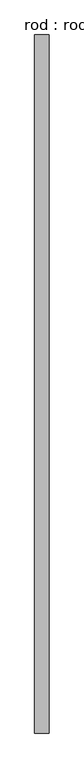
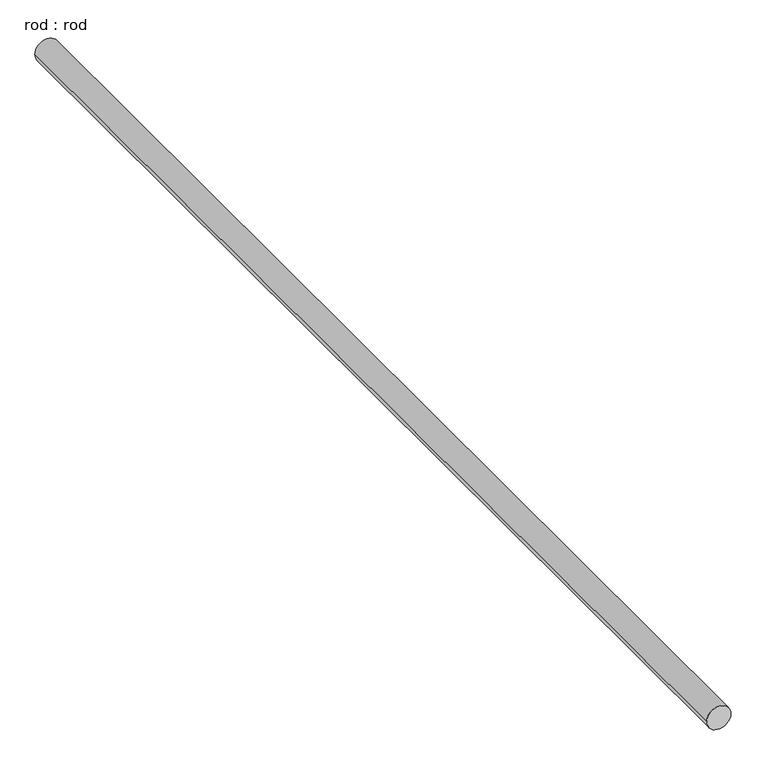
"""IFC4 building model written with IfcOpenShell, lengths in millimetres: proxy geometry, rod : rod."""

from ifc_helpers import new_model, si_unit, point, frame, frame_2d, origin, place, context, project, spatial, circle_curve, trimmed, segment, composite_curve, outline, extrude, source, transform, mapped, element, save


def rod_rod_0f7073d6(model_context):
    return source(origin(), model_context, "Body", "SweptSolid", [
        extrude(outline(composite_curve([segment(trimmed(circle_curve(frame_2d((0.0108462, 0.0)), 200.0), [point((0.0108462, 200.0))], [point((0.0108462, -200.0))], False, "CARTESIAN"), True, "CONTINUOUS"), segment(trimmed(circle_curve(frame_2d((0.0108462, 0.0)), 200.0), [point((0.0108462, -200.0))], [point((0.0108462, 200.0))], False, "CARTESIAN"), True, "CONTINUOUS")], self_intersect=False)), frame((0.0, -5536.7356704, 0.0), z_axis=(0.0, 1.0, 0.0), x_axis=(0.0, 0.0, 1.0)), (0.0, 0.0, 1.0), 19258.9285714),
    ])


if __name__ == "__main__":
    model = new_model("IFC4")
    model_context = context("Model", 3, world=origin())
    ifc_project = project(units=[si_unit("LENGTHUNIT", "METRE", prefix="MILLI")], contexts=[model_context])
    site = spatial("IfcSite", under=ifc_project)
    building = spatial("IfcBuilding", under=site)
    placement = place(None, origin())
    rod_rod_shape = rod_rod_0f7073d6(model_context)
    element("IfcBuildingElementProxy", 1, Name="rod : rod", ObjectType="rod : rod", at=placement, inside=building, context=model_context, shape_type="MappedRepresentation", body=[
        mapped(rod_rod_shape, transform((0.0, 0.0, 0.0), x_axis=(1.0, 0.0, 0.0), y_axis=(0.0, 1.0, 0.0), z_axis=(0.0, 0.0, 1.0))),
    ])
    save(model, "model.ifc")

# Revit data of these elements
# Type "rod : rod"
#   Default Elevation = 0
